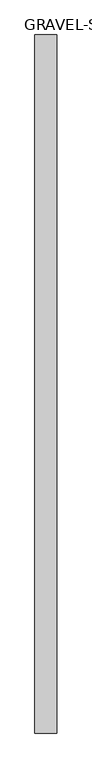
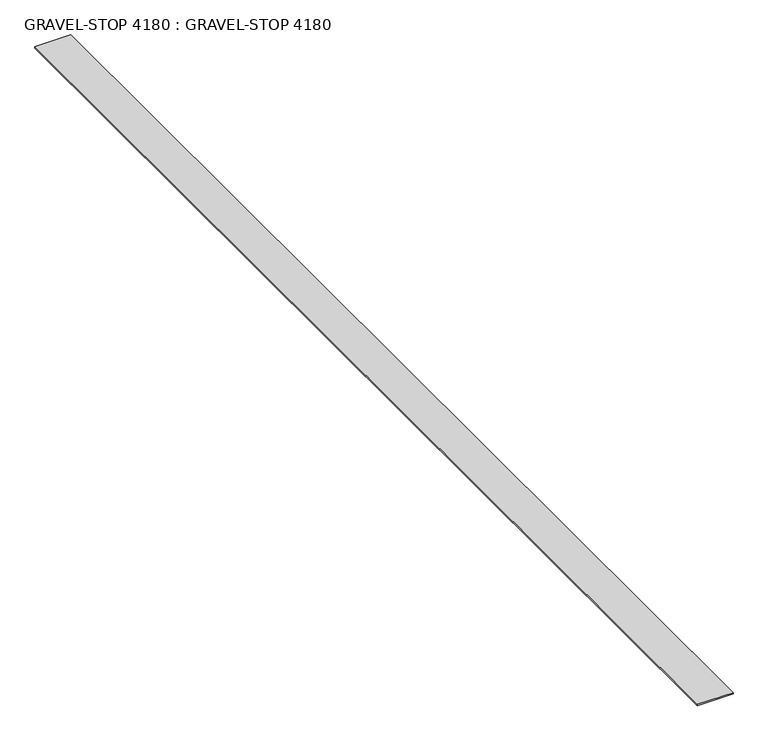
"""IFC4 building model written with IfcOpenShell, lengths in millimetres: proxy geometry, GRAVEL-STOP 4180 : GRAVEL-STOP 4180."""

from ifc_helpers import new_model, si_unit, frame, origin, place, context, project, spatial, polyline, outline, extrude, source, transform, mapped, element, save


def gravel_stop_4180_gravel_stop_4180_df2d17d1(model_context):
    return source(origin(), model_context, "Body", "SweptSolid", [
        extrude(outline(polyline([(-2737.5325942, 947.3593427), (-2675.2044862, 947.3593427), (-2675.2044862, -1052.8906573), (-2737.5325942, -1052.8906573), (-2737.5325942, 947.3593427)])), frame((0.0, 0.0, 40252.8572765), z_axis=(0.0, 0.0, 1.0), x_axis=(1.0, 0.0, 0.0)), (0.0, 0.0, 1.0), 2.3397091),
    ])


if __name__ == "__main__":
    model = new_model("IFC4")
    model_context = context("Model", 3, world=origin())
    ifc_project = project(units=[si_unit("LENGTHUNIT", "METRE", prefix="MILLI")], contexts=[model_context])
    site = spatial("IfcSite", under=ifc_project)
    building = spatial("IfcBuilding", under=site)
    placement = place(None, origin())
    gravel_stop_4180_gravel_stop_4180_shape = gravel_stop_4180_gravel_stop_4180_df2d17d1(model_context)
    element("IfcBuildingElementProxy", 1, Name="GRAVEL-STOP 4180 : GRAVEL-STOP 4180", ObjectType="GRAVEL-STOP 4180 : GRAVEL-STOP 4180", at=placement, inside=building, context=model_context, shape_type="MappedRepresentation", body=[
        mapped(gravel_stop_4180_gravel_stop_4180_shape, transform((0.0, 0.0, 0.0), x_axis=(1.0, 0.0, 0.0), y_axis=(0.0, 1.0, 0.0), z_axis=(0.0, 0.0, 1.0))),
    ])
    save(model, "model.ifc")

# Revit data of these elements
# Type "GRAVEL-STOP 4180 : GRAVEL-STOP 4180"
#   NameOverride = "GRAVEL-STOP"
# Element 1 (IfcBuildingElementProxy, "GRAVEL-STOP 4180 : GRAVEL-STOP 4180")
#   Materials on its faces: "METAL FLASHING"
# Materials
#   "METAL FLASHING": class "Unassigned", colour RGB 128 128 128, transparency 0
